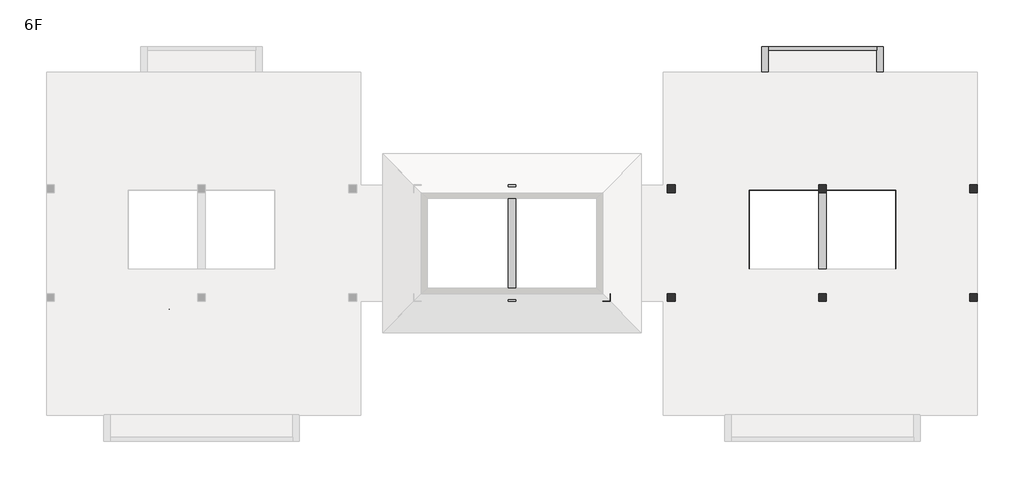
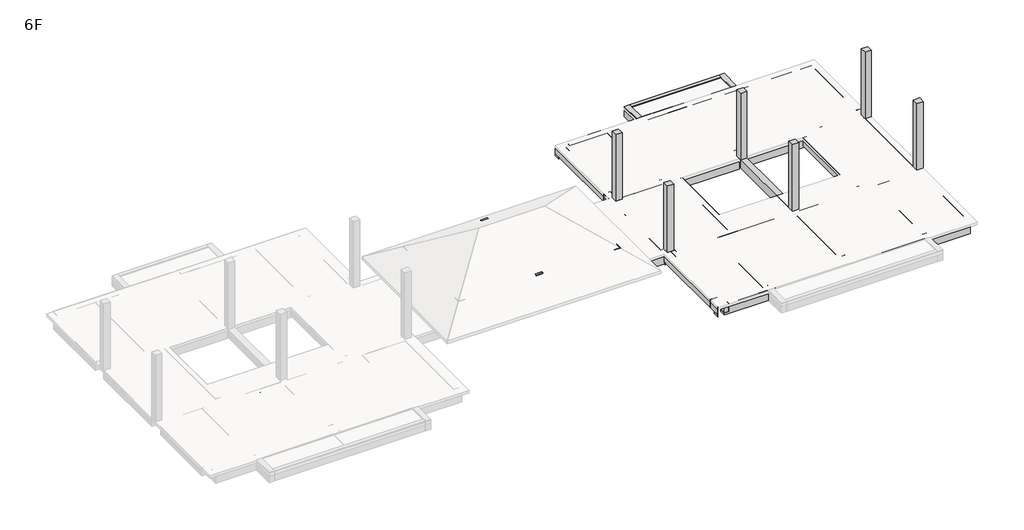
# One storey, part 2 of 2: 33 beams, 10 columns, 1 proxy.
"""IFC4 building model written with IfcOpenShell, lengths in millimetres."""

import ifcopenshell
import ifcopenshell.guid

model = None  # the IFC model being written
_history = None  # IfcOwnerHistory: only IFC2X3 demands one
_inside = {}  # id of a spatial element -> (the spatial element, [elements in it])
_under = {}  # id of a project, library or spatial element -> (it, [spatial elements below it])
_declared = {}  # id of a project -> (the project, [libraries it declares])
_typed = {}  # id of a type object -> (the type object, [elements of that type])
_made_of = {}  # id of a material, layer set ... -> (it, [elements and type objects made of it])


def new_model(schema):
    """Start an empty IFC model of exactly this schema.

    Asked for "IFC4X3", IfcOpenShell would pick the latest addendum, in which some entities
    have other attributes; the version numbers below select the first issue.
    IFC2X3 requires an IfcOwnerHistory on every rooted entity: one is made here for all.
    """
    global model, _history
    if schema == "IFC4X3":
        model = ifcopenshell.file(schema_version=(4, 3, 0, 0))
    else:
        model = ifcopenshell.file(schema=schema)
    _inside.clear()
    _under.clear()
    _declared.clear()
    _typed.clear()
    _made_of.clear()
    _history = None
    if model.schema == "IFC2X3":
        org = make("IfcOrganization", Name="unknown")
        user = make(
            "IfcPersonAndOrganization",
            ThePerson=make("IfcPerson", FamilyName="unknown"),
            TheOrganization=org,
        )
        app = make(
            "IfcApplication",
            ApplicationDeveloper=org,
            Version="unknown",
            ApplicationFullName="unknown",
            ApplicationIdentifier="unknown",
        )
        _history = make(
            "IfcOwnerHistory",
            OwningUser=user,
            OwningApplication=app,
            ChangeAction="ADDED",
            CreationDate=0,
        )
    return model


def make(cls, **values):
    """One entity of the class cls with the attributes given. An attribute that is None is left unset."""
    return model.create_entity(
        cls, **{name: value for name, value in values.items() if value is not None}
    )


def rooted(cls, **values):
    """An entity with a GlobalId (a new one), such as an element, a storey or a relation."""
    return make(cls, GlobalId=ifcopenshell.guid.new(), OwnerHistory=_history, **values)


def si_unit(unit_type, name, prefix=None):
    """IfcSIUnit, for example si_unit("LENGTHUNIT", "METRE", prefix="MILLI")."""
    return make("IfcSIUnit", UnitType=unit_type, Prefix=prefix, Name=name)


def assignment(units):
    """IfcUnitAssignment: the units of a project."""
    return None if units is None else make("IfcUnitAssignment", Units=units)


def point(xyz):
    """IfcCartesianPoint."""
    return None if xyz is None else make("IfcCartesianPoint", Coordinates=xyz)


def direction(xyz):
    """IfcDirection."""
    return None if xyz is None else make("IfcDirection", DirectionRatios=xyz)


def frame(location, z_axis=None, x_axis=None):
    """IfcAxis2Placement3D, a coordinate frame: its origin and axes. An axis left out is left unset."""
    return make(
        "IfcAxis2Placement3D",
        Location=point(location),
        Axis=direction(z_axis),
        RefDirection=direction(x_axis),
    )


def frame_2d(location, x_axis=None):
    """IfcAxis2Placement2D, a coordinate frame in the plane: its origin and x axis."""
    return make(
        "IfcAxis2Placement2D", Location=point(location), RefDirection=direction(x_axis)
    )


def origin():
    """The frame at (0, 0, 0) with its axes left unset."""
    return frame((0.0, 0.0, 0.0))


def origin_with_axes():
    """The frame at (0, 0, 0) with the z axis (0, 0, 1) and the x axis (1, 0, 0) written out."""
    return frame((0.0, 0.0, 0.0), z_axis=(0.0, 0.0, 1.0), x_axis=(1.0, 0.0, 0.0))


def place(relative_to, where):
    """IfcLocalPlacement: puts the frame where relative to a parent placement (None: the world)."""
    return make(
        "IfcLocalPlacement", PlacementRelTo=relative_to, RelativePlacement=where
    )


def context(
    kind, dimensions, precision=None, world=None, true_north=None, identifier=None
):
    """IfcGeometricRepresentationContext, for example the 3D "Model" context."""
    return make(
        "IfcGeometricRepresentationContext",
        ContextIdentifier=identifier,
        ContextType=kind,
        CoordinateSpaceDimension=dimensions,
        Precision=precision,
        WorldCoordinateSystem=world,
        TrueNorth=true_north,
    )


def project(units=None, contexts=None):
    """IfcProject with its units and contexts."""
    return rooted(
        "IfcProject",
        Name="project",
        RepresentationContexts=contexts,
        UnitsInContext=assignment(units),
    )


def spatial(cls, under=None, at=None, **own):
    """A site, building, storey or space (cls), placed at a placement, below another one or the project."""
    s = rooted(cls, ObjectPlacement=at, **own)
    if under is not None:
        _under.setdefault(under.id(), (under, []))[1].append(s)
    return s


def polyline(points):
    """IfcPolyline through the points."""
    return make("IfcPolyline", Points=[point(p) for p in points])


def circle_curve(where, radius):
    """IfcCircle in the frame where."""
    return make("IfcCircle", Position=where, Radius=radius)


def ellipse_curve(where, semi_axis1, semi_axis2):
    """IfcEllipse in the frame where."""
    return make(
        "IfcEllipse", Position=where, SemiAxis1=semi_axis1, SemiAxis2=semi_axis2
    )


def trimmed(basis, trim1, trim2, sense, master):
    """IfcTrimmedCurve: the piece of a basis curve between two trims."""
    return make(
        "IfcTrimmedCurve",
        BasisCurve=basis,
        Trim1=trim1,
        Trim2=trim2,
        SenseAgreement=sense,
        MasterRepresentation=master,
    )


def segment(curve, same_sense, transition):
    """IfcCompositeCurveSegment."""
    return make(
        "IfcCompositeCurveSegment",
        Transition=transition,
        SameSense=same_sense,
        ParentCurve=curve,
    )


def composite_curve(segments, self_intersect=None):
    """IfcCompositeCurve: segments joined end to end."""
    return make("IfcCompositeCurve", Segments=segments, SelfIntersect=self_intersect)


def outline(outer, holes=None, kind="AREA"):
    """IfcArbitraryClosedProfileDef: a profile drawn as a closed curve; with holes, ...WithVoids."""
    if holes is None:
        return make("IfcArbitraryClosedProfileDef", ProfileType=kind, OuterCurve=outer)
    return make(
        "IfcArbitraryProfileDefWithVoids",
        ProfileType=kind,
        OuterCurve=outer,
        InnerCurves=holes,
    )


def extrude(swept, where, along, depth):
    """IfcExtrudedAreaSolid: the profile swept, set in the frame where, extruded along a direction by depth."""
    return make(
        "IfcExtrudedAreaSolid",
        SweptArea=swept,
        Position=where,
        ExtrudedDirection=direction(along),
        Depth=depth,
    )


def faces_of(points, faces, orient=None, outer=None):
    """IfcFace entities. A face is a list of loops; a loop is a list of indices into points, from 0.

    orient and outer hold one flag for each loop. By default every Orientation is true, the
    first loop of a face is its IfcFaceOuterBound and the others are IfcFaceBound.
    """
    made = []
    for i, loops in enumerate(faces):
        bounds = []
        for j, loop in enumerate(loops):
            is_outer = j == 0 if outer is None else outer[i][j]
            bounds.append(
                make(
                    "IfcFaceOuterBound" if is_outer else "IfcFaceBound",
                    Bound=make("IfcPolyLoop", Polygon=[points[k] for k in loop]),
                    Orientation=True if orient is None else orient[i][j],
                )
            )
        made.append(make("IfcFace", Bounds=bounds))
    return made


def faceted_brep(points, faces, orient=None, outer=None, voids=None):
    """IfcFacetedBrep: a solid bounded by flat faces; with voids (closed shells), ...WithVoids."""
    shared = [point(p) for p in points]
    hull = make("IfcClosedShell", CfsFaces=faces_of(shared, faces, orient, outer))
    if voids is None:
        return make("IfcFacetedBrep", Outer=hull)
    return make(
        "IfcFacetedBrepWithVoids",
        Outer=hull,
        Voids=[
            make(cls, CfsFaces=faces_of(shared, fs, o, b)) for cls, fs, o, b in voids
        ],
    )


def shape(context_of_items, identifier, shape_type, items):
    """IfcShapeRepresentation: the items that make up one representation, for example the "Body"."""
    return make(
        "IfcShapeRepresentation",
        ContextOfItems=context_of_items,
        RepresentationIdentifier=identifier,
        RepresentationType=shape_type,
        Items=items,
    )


def source(mapping_origin, context_of_items, identifier, shape_type, items):
    """IfcRepresentationMap: a shape defined once, which mapped items show again and again."""
    return make(
        "IfcRepresentationMap",
        MappingOrigin=mapping_origin,
        MappedRepresentation=shape(context_of_items, identifier, shape_type, items),
    )


def transform(
    local_origin,
    x_axis=None,
    y_axis=None,
    z_axis=None,
    scale=None,
    scale2=None,
    scale3=None,
    uniform=True,
):
    """IfcCartesianTransformationOperator3D, or its non-uniform kind. x_axis, y_axis, z_axis: its Axis1, 2, 3."""
    if uniform:
        return make(
            "IfcCartesianTransformationOperator3D",
            Axis1=direction(x_axis),
            Axis2=direction(y_axis),
            LocalOrigin=point(local_origin),
            Scale=scale,
            Axis3=direction(z_axis),
        )
    return make(
        "IfcCartesianTransformationOperator3DnonUniform",
        Axis1=direction(x_axis),
        Axis2=direction(y_axis),
        LocalOrigin=point(local_origin),
        Scale=scale,
        Axis3=direction(z_axis),
        Scale2=scale2,
        Scale3=scale3,
    )


def mapped(mapping_source, mapping_target):
    """IfcMappedItem: shows the shape of a source again, moved by a transform."""
    return make(
        "IfcMappedItem", MappingSource=mapping_source, MappingTarget=mapping_target
    )


def made_of(thing, what):
    """Note that an element or type object is made of a material, layer set ...; save() writes the relation."""
    if what is not None:
        _made_of.setdefault(what.id(), (what, []))[1].append(thing)
    return thing


def element(
    cls,
    number,
    at=None,
    inside=None,
    cuts=None,
    type_object=None,
    material=None,
    context=None,
    identifier="Body",
    shape_type=None,
    held_by="IfcProductDefinitionShape",
    body=None,
    shapes=None,
    **own,
):
    """One element of the class cls, such as IfcWall. Its Tag is "e" and its number.

    at: its placement. inside: the storey or other place that contains it. cuts: it is an
    opening in that element (IfcRelVoidsElement). A single representation is given by context,
    identifier, shape_type and body (its items); several are given by shapes. held_by: the class
    of the entity that holds the representations. save() writes the other relations.
    """
    e = rooted(cls, Tag="e%d" % number, ObjectPlacement=at, **own)
    if body is not None:
        shapes = [shape(context, identifier, shape_type, body)]
    if shapes is not None:
        e.Representation = make(held_by, Representations=shapes)
    if inside is not None:
        _inside.setdefault(inside.id(), (inside, []))[1].append(e)
    if cuts is not None:
        rooted(
            "IfcRelVoidsElement", RelatingBuildingElement=cuts, RelatedOpeningElement=e
        )
    if type_object is not None:
        _typed.setdefault(type_object.id(), (type_object, []))[1].append(e)
    return made_of(e, material)


def aggregate(whole, parts):
    """IfcRelAggregates: a whole, such as a stair, and the parts it consists of."""
    return rooted("IfcRelAggregates", RelatingObject=whole, RelatedObjects=parts)


def save(model, path):
    """Write the relations noted so far, then the file.

    IfcRelAggregates (storeys below a building ...), IfcRelContainedInSpatialStructure (elements
    in a storey), IfcRelDefinesByType, IfcRelAssociatesMaterial and IfcRelDeclares: one each for
    every whole, place, type object, material and project.
    """
    for whole, parts in _under.values():
        aggregate(whole, parts)
    for where, things in _inside.values():
        rooted(
            "IfcRelContainedInSpatialStructure",
            RelatedElements=things,
            RelatingStructure=where,
        )
    for kind, things in _typed.values():
        rooted("IfcRelDefinesByType", RelatedObjects=things, RelatingType=kind)
    for what, things in _made_of.values():
        rooted("IfcRelAssociatesMaterial", RelatedObjects=things, RelatingMaterial=what)
    for by, libraries in _declared.values():
        rooted("IfcRelDeclares", RelatingContext=by, RelatedDefinitions=libraries)
    model.write(path)


def plane_surface(at):
    """IfcPlane: the flat surface through the origin of the frame at, square to its z axis."""
    return make("IfcPlane", Position=at)


def cylinder_surface(at, radius):
    """IfcCylindricalSurface: all points at the distance radius from the z axis of the frame at."""
    return make("IfcCylindricalSurface", Position=at, Radius=radius)


def revolved_surface(curve, axis_point, axis_direction):
    """IfcSurfaceOfRevolution: the curve turned about the line through axis_point along axis_direction."""
    return make(
        "IfcSurfaceOfRevolution",
        SweptCurve=make("IfcArbitraryOpenProfileDef", ProfileType="CURVE", Curve=curve),
        AxisPosition=make("IfcAxis1Placement", Location=point(axis_point), Axis=direction(axis_direction)),
    )


def advanced_brep(points, edges, surfaces, faces):
    """IfcAdvancedBrep: a solid bounded by faces that lie on surfaces and meet in shared edges.

    An edge is (start, end): straight between two places in points (the first is 0);
    or (start, end, curve); or (start, end, curve, False) where it runs against its curve.
    A face is (place in surfaces, loops), or (place, loops, False) where it looks against
    its surface's normal. A loop lists edges by number (the first is 1), with a minus sign
    where the edge is run from its end to its start. The first loop is the outer one.
    """
    corners = [point(p) for p in points]
    vertices = [make("IfcVertexPoint", VertexGeometry=c) for c in corners]
    made = []
    for start, end, *more in edges:
        made.append(
            make(
                "IfcEdgeCurve",
                EdgeStart=vertices[start],
                EdgeEnd=vertices[end],
                EdgeGeometry=more[0] if more else make("IfcPolyline", Points=[corners[start], corners[end]]),
                SameSense=more[1] if len(more) > 1 else True,
            )
        )
    hull = []
    for where, loops, *sense in faces:
        bounds = []
        for j, loop in enumerate(loops):
            ring = [make("IfcOrientedEdge", EdgeElement=made[abs(k) - 1], Orientation=k > 0) for k in loop]
            bounds.append(
                make(
                    "IfcFaceOuterBound" if j == 0 else "IfcFaceBound",
                    Bound=make("IfcEdgeLoop", EdgeList=ring),
                    Orientation=True,
                )
            )
        hull.append(make("IfcAdvancedFace", Bounds=bounds, FaceSurface=surfaces[where], SameSense=sense[0] if sense else True))
    return make("IfcAdvancedBrep", Outer=make("IfcClosedShell", CfsFaces=hull))


def m_support_metal_circular_m_support_metal_circular_a779fbb7(model_context):
    return source(origin(), model_context, "Body", "SolidModel", [
        advanced_brep(
        [(-6.0, 0.0, 0.0), (6.0, 0.0, 0.0), (-6.0, 0.0, -63.0), (6.0, 0.0, -63.0), (6.0, 12.0, -75.0), (-6.0, 12.0, -75.0), (-6.0, 63.0, -75.0), (6.0, 63.0, -75.0)],
        [
            (0, 1, circle_curve(origin_with_axes(), 6.0)),
            (1, 0, circle_curve(origin_with_axes(), 6.0)),
            (0, 2),
            (2, 3, circle_curve(frame((0.0, 0.0, -63.0), z_axis=(0.0, 0.0, 1.0), x_axis=(1.0, 0.0, 0.0)), 6.0)),
            (3, 1),
            (3, 2, circle_curve(frame((0.0, 0.0, -63.0), z_axis=(0.0, 0.0, 1.0), x_axis=(1.0, 0.0, 0.0)), 6.0)),
            (4, 3, circle_curve(frame((6.0, 12.0, -63.0), z_axis=(-1.0, 0.0, 0.0), x_axis=(0.0, -1.0, 0.0)), 12.0)),
            (2, 5, circle_curve(frame((-6.0, 12.0, -63.0), z_axis=(1.0, 0.0, 0.0), x_axis=(0.0, -1.0, 0.0)), 12.0)),
            (5, 4, circle_curve(frame((0.0, 12.0, -75.0), z_axis=(0.0, -1.0, 0.0), x_axis=(1.0, 0.0, 0.0)), 6.0)),
            (4, 5, circle_curve(frame((0.0, 12.0, -75.0), z_axis=(0.0, -1.0, 0.0), x_axis=(1.0, 0.0, 0.0)), 6.0)),
            (6, 7, circle_curve(frame((0.0, 63.0, -75.0), z_axis=(0.0, 1.0, 0.0), x_axis=(1.0, 0.0, 0.0)), 6.0)),
            (7, 6, circle_curve(frame((0.0, 63.0, -75.0), z_axis=(0.0, 1.0, 0.0), x_axis=(1.0, 0.0, 0.0)), 6.0)),
            (5, 6),
            (7, 4),
        ],
        [
            plane_surface(origin_with_axes()),
            cylinder_surface(origin_with_axes(), 6.0),
            revolved_surface(trimmed(ellipse_curve(frame((0.0, 0.0, -63.0), z_axis=(0.0, 0.0, 1.0), x_axis=(1.0, 0.0, 0.0)), 6.0, 6.0), [point((-6.0, 0.0, -63.0))], [point((6.0, 0.0, -63.0))], True, "CARTESIAN"), (0.0, 12.0, -63.0), (1.0, 0.0, 0.0)),
            revolved_surface(trimmed(ellipse_curve(frame((0.0, 0.0, -63.0), z_axis=(0.0, 0.0, 1.0), x_axis=(1.0, 0.0, 0.0)), 6.0, 6.0), [point((6.0, 0.0, -63.0))], [point((-6.0, 0.0, -63.0))], True, "CARTESIAN"), (0.0, 12.0, -63.0), (1.0, 0.0, 0.0)),
            plane_surface(frame((0.0, 63.0, -75.0), z_axis=(0.0, 1.0, 0.0), x_axis=(1.0, 0.0, 0.0))),
            cylinder_surface(frame((0.0, 12.0, -75.0), z_axis=(0.0, -1.0, 0.0), x_axis=(1.0, 0.0, 0.0)), 6.0),
        ],
        [
            (0, [[1, 2]]),
            (1, [[-1, 3, 4, 5]]),
            (1, [[-2, -5, 6, -3]]),
            (2, [[7, -4, 8, 9]]),
            (3, [[-8, -6, -7, 10]]),
            (4, [[11, 12]]),
            (5, [[-9, 13, -12, 14]]),
            (5, [[-10, -14, -11, -13]]),
        ],
    ),
        extrude(outline(composite_curve([segment(trimmed(circle_curve(frame_2d((-75.0, 0.0)), 25.0), [point((-75.0, -25.0))], [point((-75.0, 25.0))], False, "CARTESIAN"), True, "CONTINUOUS"), segment(trimmed(circle_curve(frame_2d((-75.0, 0.0)), 25.0), [point((-75.0, 25.0))], [point((-75.0, -25.0))], False, "CARTESIAN"), True, "CONTINUOUS")], self_intersect=False)), frame((0.0, 63.0, 0.0), z_axis=(0.0, 1.0, 0.0), x_axis=(0.0, 0.0, 1.0)), (0.0, 0.0, 1.0), 12.0),
    ])


model = new_model("IFC4")

# Units and contexts
model_context = context("Model", 3, world=origin())
ifc_project = project(units=[si_unit("LENGTHUNIT", "METRE", prefix="MILLI")], contexts=[model_context])

# Site, building, storey
site = spatial("IfcSite", under=ifc_project)
building = spatial("IfcBuilding", under=site)
storey = spatial("IfcBuildingStorey", under=building, Name="6F", Elevation=17230.0)

# Beams
placement = place(None, origin())
element("IfcBeam", 1, ObjectType="M_Concrete-Rectangular Beam : 150x500", at=placement, inside=storey, context=model_context, shape_type="SweptSolid", body=[
    extrude(outline(polyline([(31939.6333637, 14100.0000002), (31939.6333637, 13950.0000002), (27759.4337113, 13950.0000002), (27759.4337113, 14100.0000002), (31939.6333637, 14100.0000002)])), frame((0.0, 0.0, 16730.0), z_axis=(0.0, 0.0, 1.0), x_axis=(1.0, 0.0, 0.0)), (0.0, 0.0, 1.0), 500.0),
])
element("IfcBeam", 2, ObjectType="M_Concrete-Rectangular Beam : 250x400", at=placement, inside=storey, context=model_context, shape_type="Brep", body=[
    faceted_brep([(32930.0000108, 8549.9999993, 17230.0), (32680.0000108, 8549.9999993, 17230.0), (32680.0000108, 4449.9999998, 17230.0), (32930.0000108, 4449.9999998, 17230.0), (32930.0000108, 8549.9999993, 16830.0), (32930.0000108, 4449.9999998, 16830.0), (32680.0000108, 8549.9999993, 16830.0), (32680.0000108, 4449.9999998, 16830.0), (32680.0000108, 8549.9999993, 17088.8582284)], [[[0, 1, 2, 3]], [[4, 0, 3, 5]], [[6, 4, 5, 7]], [[1, 8, 6, 7, 2]], [[1, 0, 4, 6, 8]], [[3, 2, 7, 5]]]),
])
element("IfcBeam", 3, ObjectType="M_Concrete-Rectangular Beam : 250x400", at=placement, inside=storey, context=model_context, shape_type="SweptSolid", body=[
    extrude(outline(polyline([(21399.9824991, 8449.9999993), (21649.9824991, 8449.9999993), (21649.9824991, 4549.9999902), (21399.9824991, 4549.9999902), (21399.9824991, 8449.9999993)])), frame((0.0, 0.0, 16830.0), z_axis=(0.0, 0.0, 1.0), x_axis=(1.0, 0.0, 0.0)), (0.0, 0.0, 1.0), 400.0),
])
element("IfcBeam", 4, ObjectType="M_Concrete-Rectangular Beam : 250x400", at=placement, inside=storey, context=model_context, shape_type="Brep", body=[
    faceted_brep([(27020.000004, 8549.9999993, 17230.0), (26770.000004, 8549.9999993, 17230.0), (26770.000004, 4449.9999998, 17230.0), (27020.000004, 4449.9999998, 17230.0), (27020.000004, 8549.9999993, 16830.0), (27020.000004, 8549.9999993, 17088.8582239), (27020.000004, 4449.9999998, 16830.0), (26770.000004, 8549.9999993, 16830.0), (26770.000004, 4449.9999998, 16830.0)], [[[0, 1, 2, 3]], [[4, 5, 0, 3, 6]], [[7, 4, 6, 8]], [[1, 7, 8, 2]], [[1, 0, 5, 4, 7]], [[3, 2, 8, 6]]]),
])
element("IfcBeam", 5, ObjectType="M_Concrete-Rectangular Beam : 250x400", at=placement, inside=storey, context=model_context, shape_type="SweptSolid", body=[
    extrude(outline(polyline([(25965.079965, 12800.0000001), (26215.079965, 12800.0000001), (26215.079965, 8849.9999993), (25965.079965, 8849.9999993), (25965.079965, 12800.0000001)])), frame((0.0, 0.0, 16830.0), z_axis=(0.0, 0.0, 1.0), x_axis=(1.0, 0.0, 0.0)), (0.0, 0.0, 1.0), 400.0),
])
element("IfcBeam", 6, ObjectType="M_Concrete-Rectangular Beam : 250x400", at=placement, inside=storey, context=model_context, shape_type="SweptSolid", body=[
    extrude(outline(polyline([(25965.079965, 4149.9999998), (26215.079965, 4149.9999998), (26215.079965, 199.9999987), (25965.079965, 199.9999987), (25965.079965, 4149.9999998)])), frame((0.0, 0.0, 16830.0), z_axis=(0.0, 0.0, 1.0), x_axis=(1.0, 0.0, 0.0)), (0.0, 0.0, 1.0), 400.0),
])
element("IfcBeam", 7, ObjectType="M_Concrete-Rectangular Beam : 250x400", at=placement, inside=storey, context=model_context, shape_type="SweptSolid", body=[
    extrude(outline(polyline([(33485.0000061, 12800.0000001), (33735.0000061, 12800.0000001), (33735.0000061, 8849.9999993), (33485.0000061, 8849.9999993), (33485.0000061, 12800.0000001)])), frame((0.0, 0.0, 16830.0), z_axis=(0.0, 0.0, 1.0), x_axis=(1.0, 0.0, 0.0)), (0.0, 0.0, 1.0), 400.0),
])
element("IfcBeam", 8, ObjectType="M_Concrete-Rectangular Beam : 250x400", at=placement, inside=storey, context=model_context, shape_type="SweptSolid", body=[
    extrude(outline(polyline([(33485.0000061, 4149.9999998), (33735.0000061, 4149.9999998), (33735.0000061, 199.9999987), (33485.0000061, 199.9999987), (33485.0000061, 4149.9999998)])), frame((0.0, 0.0, 16830.0), z_axis=(0.0, 0.0, 1.0), x_axis=(1.0, 0.0, 0.0)), (0.0, 0.0, 1.0), 400.0),
])
element("IfcBeam", 9, ObjectType="M_Concrete-Rectangular Beam : 250x400", at=placement, inside=storey, context=model_context, shape_type="SweptSolid", body=[
    extrude(outline(polyline([(18180.0, 21379.9824991), (17780.0, 21379.9824991), (17780.0, 21629.9824991), (18098.9682373, 21629.9824991), (18180.0, 21508.4286852), (18180.0, 21379.9824991)])), frame((0.0, 4550.0000005, 0.0), z_axis=(0.0, 1.0, 0.0), x_axis=(0.0, 0.0, 1.0)), (0.0, 0.0, 1.0), 3899.9999997),
])
element("IfcBeam", 10, ObjectType="M_Concrete-Rectangular Beam : 250x400", at=placement, inside=storey, context=model_context, shape_type="SweptSolid", body=[
    extrude(outline(polyline([(8724.9999993, 17780.0), (8474.9999993, 17780.0), (8474.9999993, 18180.0), (8608.4366337, 18180.0), (8724.9999993, 18102.2891349), (8724.9999993, 17780.0)])), frame((14350.0174936, 0.0, 0.0), z_axis=(1.0, 0.0, 0.0), x_axis=(0.0, 1.0, 0.0)), (0.0, 0.0, 1.0), 3349.7492755),
    extrude(outline(polyline([(8724.9999993, 17780.0), (8474.9999993, 17780.0), (8474.9999993, 18180.0), (8608.4366337, 18180.0), (8724.9999993, 18102.2891349), (8724.9999993, 17780.0)])), frame((17999.7667691, 0.0, 0.0), z_axis=(1.0, 0.0, 0.0), x_axis=(0.0, 1.0, 0.0)), (0.0, 0.0, 1.0), 3350.0),
])
element("IfcBeam", 11, ObjectType="M_Concrete-Rectangular Beam : 250x400", at=placement, inside=storey, context=model_context, shape_type="SweptSolid", body=[
    extrude(outline(polyline([(4524.9999902, 17780.0), (4274.9999902, 17780.0), (4274.9999902, 18102.6390219), (4391.0385385, 18180.0), (4524.9999902, 18180.0), (4524.9999902, 17780.0)])), frame((17999.7667691, 0.0, 0.0), z_axis=(1.0, 0.0, 0.0), x_axis=(0.0, 1.0, 0.0)), (0.0, 0.0, 1.0), 3350.0),
    extrude(outline(polyline([(4524.9999902, 18180.0), (4524.9999902, 17780.0), (4274.9999902, 17780.0), (4274.9999902, 18102.6390219), (4391.0385385, 18180.0), (4524.9999902, 18180.0)])), frame((14350.0174936, 0.0, 0.0), z_axis=(1.0, 0.0, 0.0), x_axis=(0.0, 1.0, 0.0)), (0.0, 0.0, 1.0), 3349.7492755),
])
element("IfcBeam", 12, ObjectType="M_Concrete-Rectangular Beam : 250x500", at=placement, inside=storey, context=model_context, shape_type="Brep", body=[
    faceted_brep([(32189.6333637, 14100.0000002, 17230.0), (31939.6333637, 14100.0000002, 17230.0), (31939.6333637, 13950.0000002, 17230.0), (31939.6333637, 13100.0000001, 17230.0), (32189.6333637, 13100.0000001, 17230.0), (31939.6333637, 14100.0000002, 16730.0), (31939.6333637, 13950.0000002, 16730.0), (31939.6333637, 13100.0000001, 16730.0), (32189.6333637, 14100.0000002, 16730.0), (32189.6333637, 13100.0000001, 16730.0)], [[[0, 1, 2, 3, 4]], [[1, 5, 6, 7, 3, 2]], [[5, 8, 9, 7, 6]], [[8, 0, 4, 9]], [[1, 0, 8, 5]], [[4, 3, 7, 9]]]),
])
element("IfcBeam", 13, ObjectType="M_Concrete-Rectangular Beam : 250x500", at=placement, inside=storey, context=model_context, shape_type="Brep", body=[
    faceted_brep([(27759.4337113, 14100.0000002, 17230.0), (27509.4337113, 14100.0000002, 17230.0), (27509.4337113, 13100.0000001, 17230.0), (27759.4337113, 13100.0000001, 17230.0), (27759.4337113, 13950.0000002, 17230.0), (27509.4337113, 14100.0000002, 16730.0), (27509.4337113, 13100.0000001, 16730.0), (27759.4337113, 14100.0000002, 16730.0), (27759.4337113, 13950.0000002, 16730.0), (27759.4337113, 13100.0000001, 16730.0)], [[[0, 1, 2, 3, 4]], [[1, 5, 6, 2]], [[5, 7, 8, 9, 6]], [[7, 0, 4, 3, 9, 8]], [[1, 0, 7, 5]], [[3, 2, 6, 9]]]),
])
element("IfcBeam", 14, ObjectType="M_Concrete-Rectangular Beam : 300x400", at=placement, inside=storey, context=model_context, shape_type="Brep", body=[
    faceted_brep([(18000.0000046, 8450.0000002, 17230.0), (17700.0000046, 8449.9999993, 17230.0), (17700.0000046, 4549.9999902, 17230.0), (18000.0000046, 4549.9999902, 17230.0), (17700.0000046, 8449.9999993, 16830.0), (17700.0000046, 4549.9999902, 16830.0), (18000.0000046, 8450.0000002, 16830.0), (18000.0000046, 4549.9999902, 16830.0)], [[[0, 1, 2, 3]], [[1, 4, 5, 2]], [[4, 6, 7, 5]], [[3, 7, 6, 0]], [[0, 6, 4, 1]], [[3, 2, 5, 7]]]),
])
element("IfcBeam", 15, ObjectType="M_Concrete-Rectangular Beam : 300x400", at=placement, inside=storey, context=model_context, shape_type="SweptSolid", body=[
    extrude(outline(polyline([(30000.0000031, 9150.0000002), (29700.0000031, 9150.0000002), (29700.0000031, 12500.0000005), (30000.0000031, 12500.0000005), (30000.0000031, 9150.0000002)])), frame((0.0, 0.0, 16830.0), z_axis=(0.0, 0.0, 1.0), x_axis=(1.0, 0.0, 0.0)), (0.0, 0.0, 1.0), 400.0),
])
element("IfcBeam", 16, ObjectType="M_Concrete-Rectangular Beam : 300x400", at=placement, inside=storey, context=model_context, shape_type="SweptSolid", body=[
    extrude(outline(polyline([(30000.0000031, 4550.0000002), (29700.0000031, 4550.0000002), (29700.0000031, 8450.0000002), (30000.0000031, 8450.0000002), (30000.0000031, 4550.0000002)])), frame((0.0, 0.0, 16830.0), z_axis=(0.0, 0.0, 1.0), x_axis=(1.0, 0.0, 0.0)), (0.0, 0.0, 1.0), 400.0),
])
element("IfcBeam", 17, ObjectType="M_Concrete-Rectangular Beam : 300x400", at=placement, inside=storey, context=model_context, shape_type="SweptSolid", body=[
    extrude(outline(polyline([(30000.0000031, 500.0), (29700.0000031, 500.0), (29700.0000031, 3850.0000002), (30000.0000031, 3850.0000002), (30000.0000031, 500.0)])), frame((0.0, 0.0, 16830.0), z_axis=(0.0, 0.0, 1.0), x_axis=(1.0, 0.0, 0.0)), (0.0, 0.0, 1.0), 400.0),
])
element("IfcBeam", 18, ObjectType="M_Concrete-Rectangular Beam : 300x400", at=placement, inside=storey, context=model_context, shape_type="SweptSolid", body=[
    extrude(outline(polyline([(35835.035019, 9150.0000002), (35535.035019, 9150.0000002), (35535.035019, 12500.0000005), (35835.035019, 12500.0000005), (35835.035019, 9150.0000002)])), frame((0.0, 0.0, 16830.0), z_axis=(0.0, 0.0, 1.0), x_axis=(1.0, 0.0, 0.0)), (0.0, 0.0, 1.0), 400.0),
])
element("IfcBeam", 19, ObjectType="M_Concrete-Rectangular Beam : 300x400", at=placement, inside=storey, context=model_context, shape_type="SweptSolid", body=[
    extrude(outline(polyline([(35835.035019, 4550.0000002), (35535.035019, 4550.0000002), (35535.035019, 8450.0000002), (35835.035019, 8450.0000002), (35835.035019, 4550.0000002)])), frame((0.0, 0.0, 16830.0), z_axis=(0.0, 0.0, 1.0), x_axis=(1.0, 0.0, 0.0)), (0.0, 0.0, 1.0), 400.0),
])
element("IfcBeam", 20, ObjectType="M_Concrete-Rectangular Beam : 300x400", at=placement, inside=storey, context=model_context, shape_type="SweptSolid", body=[
    extrude(outline(polyline([(35835.035019, 500.0), (35535.035019, 500.0), (35535.035019, 3850.0000002), (35835.035019, 3850.0000002), (35835.035019, 500.0)])), frame((0.0, 0.0, 16830.0), z_axis=(0.0, 0.0, 1.0), x_axis=(1.0, 0.0, 0.0)), (0.0, 0.0, 1.0), 400.0),
])
element("IfcBeam", 21, ObjectType="M_Concrete-Rectangular Beam : 300x500", at=placement, inside=storey, context=model_context, shape_type="Brep", body=[
    faceted_brep([(24199.5160441, 8449.9999993, 17230.0), (24199.5160441, 8549.9999993, 17230.0), (24199.5160441, 8749.9999993, 17230.0), (23999.9649972, 8749.9999993, 17230.0), (23999.9649972, 8449.9999993, 17230.0), (24199.5160441, 8449.9999993, 16730.0), (24199.5160441, 8449.9999993, 16830.0), (23999.9649972, 8449.9999993, 16730.0), (24199.5160441, 8749.9999993, 16730.0), (24199.5160441, 8549.9999993, 16730.0), (23999.9649972, 8749.9999993, 16730.0), (24199.5160441, 8749.9999993, 16830.0), (23999.9649972, 8749.9999993, 16830.0)], [[[0, 1, 2, 3, 4]], [[5, 6, 0, 4, 7]], [[8, 9, 5, 7, 10]], [[2, 11, 8, 10, 12, 3]], [[2, 1, 0, 6, 5, 9, 8, 11]], [[4, 3, 12, 10, 7]]]),
    faceted_brep([(17999.9649983, 8449.9999993, 17230.0), (17999.9649983, 8749.9999993, 17230.0), (17999.9649983, 8749.9999993, 16730.0), (17999.9649983, 8449.9999993, 16730.0), (23699.9649972, 8749.9999993, 17230.0), (23699.9649972, 8449.9999993, 17230.0), (23699.9649972, 8449.9999993, 16730.0), (23699.9649972, 8749.9999993, 16730.0), (23699.9649972, 8749.9999993, 16830.0), (21399.9824991, 8449.9999993, 17230.0), (21649.9824991, 8449.9999993, 17230.0), (23699.5160441, 8449.9999993, 17230.0), (23699.5160441, 8749.9999993, 17230.0), (23699.5160441, 8749.9999993, 16730.0)], [[[0, 1, 2, 3]], [[4, 5, 6, 7, 8]], [[1, 0, 9, 10, 11, 5, 4, 12]], [[0, 3, 6, 5, 11, 10, 9]], [[3, 2, 13, 7, 6]], [[2, 1, 12, 4, 8, 7, 13]]]),
])
element("IfcBeam", 22, ObjectType="M_Concrete-Rectangular Beam : 300x500", at=placement, inside=storey, context=model_context, shape_type="Brep", body=[
    faceted_brep([(24199.5160441, 4249.9999902, 17230.0), (24199.5160441, 4449.9999998, 17230.0), (24199.5160441, 4549.9999902, 17230.0), (24000.0000047, 4549.9999902, 17230.0), (24000.0000047, 4249.9999902, 17230.0), (24199.5160441, 4249.9999902, 16730.0), (24199.5160441, 4249.9999902, 16830.0), (24000.0000047, 4249.9999902, 16830.0), (24000.0000047, 4249.9999902, 16730.0), (24199.5160441, 4549.9999902, 16730.0), (24199.5160441, 4449.9999998, 16730.0), (24000.0000047, 4549.9999902, 16730.0), (24199.5160441, 4549.9999902, 16830.0)], [[[0, 1, 2, 3, 4]], [[5, 6, 0, 4, 7, 8]], [[9, 10, 5, 8, 11]], [[2, 12, 9, 11, 3]], [[2, 1, 0, 6, 5, 10, 9, 12]], [[4, 3, 11, 8, 7]]]),
    faceted_brep([(18000.0000058, 4249.9999902, 17230.0), (18000.0000058, 4549.9999902, 17230.0), (18000.0000058, 4549.9999902, 16730.0), (18000.0000058, 4249.9999902, 16730.0), (23700.0000047, 4549.9999902, 17230.0), (23700.0000047, 4249.9999902, 17230.0), (23700.0000047, 4249.9999902, 16830.0), (23700.0000047, 4249.9999902, 16730.0), (23700.0000047, 4549.9999902, 16730.0), (23699.5160441, 4249.9999902, 17230.0), (23699.5160441, 4549.9999902, 17230.0), (21649.9824991, 4549.9999902, 17230.0), (21399.9824991, 4549.9999902, 17230.0), (23699.5160441, 4249.9999902, 16730.0)], [[[0, 1, 2, 3]], [[4, 5, 6, 7, 8]], [[1, 0, 9, 5, 4, 10, 11, 12]], [[0, 3, 13, 7, 6, 5, 9]], [[3, 2, 8, 7, 13]], [[2, 1, 12, 11, 10, 4, 8]]]),
])
element("IfcBeam", 23, ObjectType="M_Concrete-Rectangular Beam : 300x500", at=placement, inside=storey, context=model_context, shape_type="Brep", body=[
    faceted_brep([(24199.5160441, 13100.0000001, 17230.0), (24199.5160441, 12800.0000001, 17230.0), (25965.079965, 12800.0000001, 17230.0), (26215.079965, 12800.0000001, 17230.0), (29700.0000039, 12800.0000001, 17230.0), (29700.0000039, 13100.0000001, 17230.0), (27759.4337113, 13100.0000001, 17230.0), (27509.4337113, 13100.0000001, 17230.0), (24199.5160441, 12800.0000001, 16830.0), (24000.0000047, 12800.0000001, 16830.0), (24000.0000047, 12800.0000001, 16730.0), (29700.0000039, 12800.0000001, 16730.0), (29700.0000039, 13100.0000001, 16730.0), (24000.0000047, 13100.0000001, 16730.0), (27509.4337113, 13100.0000001, 16730.0), (27759.4337113, 13100.0000001, 16730.0), (24000.0000047, 13100.0000001, 16830.0), (24199.5160441, 13100.0000001, 16830.0)], [[[0, 1, 2, 3, 4, 5, 6, 7]], [[1, 8, 9, 10, 11, 4, 3, 2]], [[12, 11, 10, 13, 14, 15]], [[5, 12, 15, 14, 13, 16, 17, 0, 7, 6]], [[8, 17, 16, 9]], [[1, 0, 17, 8]], [[5, 4, 11, 12]], [[10, 9, 16, 13]]]),
    faceted_brep([(23699.5160441, 13100.0000001, 16730.0), (23699.5160441, 12800.0000001, 16730.0), (23699.5160441, 12800.0000001, 16830.0), (23699.5160441, 13100.0000001, 16830.0), (23700.0000047, 12800.0000001, 16830.0), (23700.0000047, 12800.0000001, 16730.0), (23700.0000047, 13100.0000001, 16730.0), (23700.0000047, 13100.0000001, 16830.0)], [[[0, 1, 2, 3]], [[4, 5, 6, 7]], [[2, 1, 5, 4]], [[1, 0, 6, 5]], [[0, 3, 7, 6]], [[3, 2, 4, 7]]]),
])
element("IfcBeam", 24, ObjectType="M_Concrete-Rectangular Beam : 300x500", at=placement, inside=storey, context=model_context, shape_type="Brep", body=[
    faceted_brep([(29699.9649964, 8549.9999993, 17230.0), (29699.9649964, 8849.9999993, 17230.0), (26215.079965, 8849.9999993, 17230.0), (25965.079965, 8849.9999993, 17230.0), (24199.5160441, 8849.9999993, 17230.0), (24199.5160441, 8749.9999993, 17230.0), (24199.5160441, 8549.9999993, 17230.0), (26770.000004, 8549.9999993, 17230.0), (27020.000004, 8549.9999993, 17230.0), (29699.9649964, 8549.9999993, 16730.0), (24199.5160441, 8549.9999993, 16730.0), (29699.9649964, 8849.9999993, 16730.0), (24199.5160441, 8749.9999993, 16730.0), (23999.9649972, 8749.9999993, 16730.0), (23999.9649972, 8849.9999993, 16730.0), (23999.9649972, 8849.9999993, 16830.0), (24199.5160441, 8849.9999993, 16830.0), (23999.9649972, 8749.9999993, 16830.0), (24199.5160441, 8749.9999993, 16830.0)], [[[0, 1, 2, 3, 4, 5, 6, 7, 8]], [[9, 0, 8, 7, 6, 10]], [[11, 9, 10, 12, 13, 14]], [[1, 11, 14, 15, 16, 4, 3, 2]], [[15, 14, 13, 17]], [[4, 16, 18, 12, 10, 6, 5]], [[1, 0, 9, 11]], [[16, 15, 17, 18]], [[12, 18, 17, 13]]]),
    faceted_brep([(23699.9649972, 8849.9999993, 16830.0), (23699.5160441, 8849.9999993, 16830.0), (23699.5160441, 8749.9999993, 16830.0), (23699.9649972, 8749.9999993, 16830.0), (23699.5160441, 8849.9999993, 16730.0), (23699.5160441, 8749.9999993, 16730.0), (23699.9649972, 8849.9999993, 16730.0), (23699.9649972, 8749.9999993, 16730.0)], [[[0, 1, 2, 3]], [[1, 4, 5, 2]], [[6, 0, 3, 7]], [[4, 6, 7, 5]], [[6, 4, 1, 0]], [[3, 2, 5, 7]]]),
])
element("IfcBeam", 25, ObjectType="M_Concrete-Rectangular Beam : 300x500", at=placement, inside=storey, context=model_context, shape_type="Brep", body=[
    faceted_brep([(29700.0000039, 4149.9999998, 17230.0), (29700.0000039, 4449.9999998, 17230.0), (27020.000004, 4449.9999998, 17230.0), (26770.000004, 4449.9999998, 17230.0), (24199.5160441, 4449.9999998, 17230.0), (24199.5160441, 4249.9999902, 17230.0), (24199.5160441, 4149.9999998, 17230.0), (25965.079965, 4149.9999998, 17230.0), (26215.079965, 4149.9999998, 17230.0), (24199.5160441, 4149.9999998, 16830.0), (24000.0000047, 4149.9999998, 16830.0), (24000.0000047, 4149.9999998, 16730.0), (29700.0000039, 4149.9999998, 16730.0), (29700.0000039, 4449.9999998, 16730.0), (24000.0000047, 4249.9999902, 16730.0), (24199.5160441, 4249.9999902, 16730.0), (24199.5160441, 4449.9999998, 16730.0), (24199.5160441, 4249.9999902, 16830.0), (24000.0000047, 4249.9999902, 16830.0)], [[[0, 1, 2, 3, 4, 5, 6, 7, 8]], [[6, 9, 10, 11, 12, 0, 8, 7]], [[13, 12, 11, 14, 15, 16]], [[1, 13, 16, 4, 3, 2]], [[9, 6, 5, 4, 16, 15, 17]], [[10, 9, 17, 18]], [[11, 10, 18, 14]], [[1, 0, 12, 13]], [[17, 15, 14, 18]]]),
    faceted_brep([(23699.5160441, 4149.9999998, 16730.0), (23699.5160441, 4149.9999998, 16830.0), (23699.5160441, 4249.9999902, 16830.0), (23699.5160441, 4249.9999902, 16730.0), (23700.0000047, 4149.9999998, 16830.0), (23700.0000047, 4149.9999998, 16730.0), (23700.0000047, 4249.9999902, 16730.0), (23700.0000047, 4249.9999902, 16830.0)], [[[0, 1, 2, 3]], [[4, 5, 6, 7]], [[1, 0, 5, 4]], [[5, 0, 3, 6]], [[1, 4, 7, 2]], [[3, 2, 7, 6]]]),
])
element("IfcBeam", 26, ObjectType="M_Concrete-Rectangular Beam : 300x500", at=placement, inside=storey, context=model_context, shape_type="Brep", body=[
    faceted_brep([(24199.5160441, 199.9999987, 17230.0), (24199.5160441, -100.0000013, 17230.0), (26070.012858, -100.0000013, 17230.0), (26320.012858, -100.0000013, 17230.0), (29700.0000039, -100.0000013, 17230.0), (29700.0000039, 199.9999987, 17230.0), (26215.079965, 199.9999987, 17230.0), (25965.079965, 199.9999987, 17230.0), (24000.0000047, -100.0000013, 16830.0), (24000.0000047, -100.0000013, 16730.0), (26070.012858, -100.0000013, 16730.0), (26320.012858, -100.0000013, 16730.0), (29700.0000039, -100.0000013, 16730.0), (24199.5160441, -100.0000013, 16830.0), (24000.0000047, 199.9999987, 16730.0), (29700.0000039, 199.9999987, 16730.0), (24199.5160441, 199.9999987, 16830.0), (24000.0000047, 199.9999987, 16830.0)], [[[0, 1, 2, 3, 4, 5, 6, 7]], [[8, 9, 10, 11, 12, 4, 3, 2, 1, 13]], [[9, 14, 15, 12, 11, 10]], [[16, 0, 7, 6, 5, 15, 14, 17]], [[1, 0, 16, 13]], [[17, 8, 13, 16]], [[9, 8, 17, 14]], [[5, 4, 12, 15]]]),
    faceted_brep([(23699.5160441, 199.9999987, 16730.0), (23699.5160441, -100.0000013, 16730.0), (23699.5160441, -100.0000013, 16830.0), (23699.5160441, 199.9999987, 16830.0), (23700.0000047, -100.0000013, 16830.0), (23700.0000047, -100.0000013, 16730.0), (23700.0000047, 199.9999987, 16730.0), (23700.0000047, 199.9999987, 16830.0)], [[[0, 1, 2, 3]], [[4, 5, 6, 7]], [[2, 1, 5, 4]], [[1, 0, 6, 5]], [[0, 3, 7, 6]], [[3, 2, 4, 7]]]),
])
element("IfcBeam", 27, ObjectType="M_Concrete-Rectangular Beam : 300x500", at=placement, inside=storey, context=model_context, shape_type="Brep", body=[
    faceted_brep([(30000.0000039, 13100.0000001, 17230.0), (30000.0000039, 12800.0000001, 17230.0), (33485.0000061, 12800.0000001, 17230.0), (33735.0000061, 12800.0000001, 17230.0), (35535.035019, 12800.0000001, 17230.0), (35535.035019, 13100.0000001, 17230.0), (32189.6333637, 13100.0000001, 17230.0), (31939.6333637, 13100.0000001, 17230.0), (30000.0000039, 12800.0000001, 16730.0), (35535.035019, 12800.0000001, 16730.0), (30000.0000039, 13100.0000001, 16730.0), (31939.6333637, 13100.0000001, 16730.0), (32189.6333637, 13100.0000001, 16730.0), (35535.035019, 13100.0000001, 16730.0)], [[[0, 1, 2, 3, 4, 5, 6, 7]], [[1, 8, 9, 4, 3, 2]], [[8, 10, 11, 12, 13, 9]], [[10, 0, 7, 6, 5, 13, 12, 11]], [[1, 0, 10, 8]], [[5, 4, 9, 13]]]),
])
element("IfcBeam", 28, ObjectType="M_Concrete-Rectangular Beam : 300x500", at=placement, inside=storey, context=model_context, shape_type="Brep", body=[
    faceted_brep([(29999.9649964, 8849.9999993, 17230.0), (29999.9649964, 8549.9999993, 17230.0), (32680.0000108, 8549.9999993, 17230.0), (32930.0000108, 8549.9999993, 17230.0), (35535.0000115, 8549.9999993, 17230.0), (35535.0000115, 8849.9999993, 17230.0), (33735.0000061, 8849.9999993, 17230.0), (33485.0000061, 8849.9999993, 17230.0), (29999.9649964, 8549.9999993, 16730.0), (35535.0000115, 8549.9999993, 16730.0), (29999.9649964, 8849.9999993, 16730.0), (35535.0000115, 8849.9999993, 16730.0)], [[[0, 1, 2, 3, 4, 5, 6, 7]], [[1, 8, 9, 4, 3, 2]], [[8, 10, 11, 9]], [[10, 0, 7, 6, 5, 11]], [[1, 0, 10, 8]], [[5, 4, 9, 11]]]),
])
element("IfcBeam", 29, ObjectType="M_Concrete-Rectangular Beam : 300x500", at=placement, inside=storey, context=model_context, shape_type="Brep", body=[
    faceted_brep([(30000.0000031, 4449.9999998, 17230.0), (30000.0000031, 4149.9999998, 17230.0), (33485.0000061, 4149.9999998, 17230.0), (33735.0000061, 4149.9999998, 17230.0), (35535.035019, 4149.9999998, 17230.0), (35535.035019, 4449.9999998, 17230.0), (32930.0000108, 4449.9999998, 17230.0), (32680.0000108, 4449.9999998, 17230.0), (30000.0000039, 4149.9999998, 16730.0), (35535.035019, 4149.9999998, 16730.0), (30000.0000039, 4449.9999998, 16730.0), (35535.035019, 4449.9999998, 16730.0)], [[[0, 1, 2, 3, 4, 5, 6, 7]], [[1, 8, 9, 4, 3, 2]], [[8, 10, 11, 9]], [[10, 0, 7, 6, 5, 11]], [[1, 0, 10, 8]], [[5, 4, 9, 11]]]),
])
element("IfcBeam", 30, ObjectType="M_Concrete-Rectangular Beam : 300x500", at=placement, inside=storey, context=model_context, shape_type="Brep", body=[
    faceted_brep([(30000.0000039, 199.9999987, 17230.0), (30000.0000039, -100.0000013, 17230.0), (33380.0128581, -100.0000013, 17230.0), (33630.0128581, -100.0000013, 17230.0), (35535.035019, -100.0000013, 17230.0), (35535.035019, 199.9999987, 17230.0), (33735.0000061, 199.9999987, 17230.0), (33485.0000061, 199.9999987, 17230.0), (30000.0000039, -100.0000013, 16730.0), (33380.0128581, -100.0000013, 16730.0), (33630.0128581, -100.0000013, 16730.0), (35535.035019, -100.0000013, 16730.0), (30000.0000039, 199.9999987, 16730.0), (35535.035019, 199.9999987, 16730.0)], [[[0, 1, 2, 3, 4, 5, 6, 7]], [[1, 8, 9, 10, 11, 4, 3, 2]], [[8, 12, 13, 11, 10, 9]], [[12, 0, 7, 6, 5, 13]], [[1, 0, 12, 8]], [[5, 4, 11, 13]]]),
])
element("IfcBeam", 31, ObjectType="M_Concrete-Rectangular Beam : 500x400", at=placement, inside=storey, context=model_context, shape_type="Brep", body=[
    faceted_brep([(23999.9649972, 9150.0000002, 17230.0), (23999.9649972, 8749.9999993, 17230.0), (24199.5160441, 8749.9999993, 17230.0), (24199.5160441, 8849.9999993, 17230.0), (24199.5160441, 12800.0000001, 17230.0), (24199.5160441, 13100.0000001, 17230.0), (24000.0000047, 13100.0000001, 17230.0), (24000.0000047, 12500.0000005, 17230.0), (23700.0000047, 12500.0000005, 17230.0), (23700.0000047, 13100.0000001, 17230.0), (23699.5160441, 13100.0000001, 17230.0), (23699.5160441, 8749.9999993, 17230.0), (23699.9649972, 8749.9999993, 17230.0), (23699.9649972, 9150.0000002, 17230.0), (23699.5160441, 8749.9999993, 16830.0), (23699.5160441, 13100.0000001, 16830.0), (23699.5160441, 12800.0000001, 16830.0), (23699.5160441, 8849.9999993, 16830.0), (23999.9649972, 8749.9999993, 16830.0), (23999.9649972, 8849.9999993, 16830.0), (23999.9649972, 9150.0000002, 16830.0), (23699.9649972, 9150.0000002, 16830.0), (23699.9649972, 8849.9999993, 16830.0), (23699.9649972, 8749.9999993, 16830.0), (23700.0000047, 13100.0000001, 16830.0), (23700.0000047, 12800.0000001, 16830.0), (23700.0000047, 12500.0000005, 16830.0), (24000.0000047, 12500.0000005, 16830.0), (24000.0000047, 12800.0000001, 16830.0), (24000.0000047, 13100.0000001, 16830.0), (24199.5160441, 13100.0000001, 16830.0), (24199.5160441, 12800.0000001, 16830.0), (24199.5160441, 8849.9999993, 16830.0), (24199.5160441, 8749.9999993, 16830.0)], [[[0, 1, 2, 3, 4, 5, 6, 7, 8, 9, 10, 11, 12, 13]], [[14, 11, 10, 15, 16, 17]], [[18, 19, 20, 21, 22, 23, 14, 17, 16, 15, 24, 25, 26, 27, 28, 29, 30, 31, 32, 33]], [[30, 5, 4, 3, 2, 33, 32, 31]], [[33, 2, 1, 18]], [[0, 20, 19, 18, 1]], [[21, 13, 12, 23, 22]], [[13, 21, 20, 0]], [[27, 7, 6, 29, 28]], [[7, 27, 26, 8]], [[8, 26, 25, 24, 9]], [[15, 10, 9, 24]], [[11, 14, 23, 12]], [[5, 30, 29, 6]]]),
])
element("IfcBeam", 32, ObjectType="M_Concrete-Rectangular Beam : 500x400", at=placement, inside=storey, context=model_context, shape_type="Brep", body=[
    faceted_brep([(24000.0000047, 500.0, 17230.0), (24000.0000047, -100.0000013, 17230.0), (24199.5160441, -100.0000013, 17230.0), (24199.5160441, 199.9999987, 17230.0), (24199.5160441, 4149.9999998, 17230.0), (24199.5160441, 4249.9999902, 17230.0), (24000.0000047, 4249.9999902, 17230.0), (24000.0000047, 3850.0000002, 17230.0), (23700.0000047, 3850.0000002, 17230.0), (23700.0000047, 4249.9999902, 17230.0), (23699.5160441, 4249.9999902, 17230.0), (23699.5160441, -100.0000013, 17230.0), (23700.0000047, -100.0000013, 17230.0), (23700.0000047, 500.0, 17230.0), (24199.5160441, -100.0000013, 16830.0), (24199.5160441, 199.9999987, 16830.0), (24199.5160441, 4149.9999998, 16830.0), (24199.5160441, 4249.9999902, 16830.0), (24000.0000047, -100.0000013, 16830.0), (24000.0000047, 199.9999987, 16830.0), (24000.0000047, 500.0, 16830.0), (23700.0000047, 500.0, 16830.0), (23700.0000047, 199.9999987, 16830.0), (23700.0000047, -100.0000013, 16830.0), (23699.5160441, -100.0000013, 16830.0), (23699.5160441, 199.9999987, 16830.0), (23699.5160441, 4149.9999998, 16830.0), (23699.5160441, 4249.9999902, 16830.0), (23700.0000047, 4249.9999902, 16830.0), (23700.0000047, 4149.9999998, 16830.0), (23700.0000047, 3850.0000002, 16830.0), (24000.0000047, 3850.0000002, 16830.0), (24000.0000047, 4149.9999998, 16830.0), (24000.0000047, 4249.9999902, 16830.0)], [[[0, 1, 2, 3, 4, 5, 6, 7, 8, 9, 10, 11, 12, 13]], [[2, 14, 15, 16, 17, 5, 4, 3]], [[18, 19, 20, 21, 22, 23, 24, 25, 26, 27, 28, 29, 30, 31, 32, 33, 17, 16, 15, 14]], [[10, 27, 26, 25, 24, 11]], [[5, 17, 33, 6]], [[0, 20, 19, 18, 1]], [[21, 13, 12, 23, 22]], [[20, 0, 13, 21]], [[31, 7, 6, 33, 32]], [[7, 31, 30, 8]], [[8, 30, 29, 28, 9]], [[11, 24, 23, 12]], [[27, 10, 9, 28]], [[14, 2, 1, 18]]]),
])
element("IfcBeam", 33, ObjectType="M_Concrete-Rectangular Beam : 500x400", at=placement, inside=storey, context=model_context, shape_type="Brep", body=[
    faceted_brep([(23699.5160441, 8449.9999993, 17230.0), (23699.5160441, 8449.9999993, 16830.0), (23699.5160441, 4549.9999902, 16830.0), (23699.5160441, 4549.9999902, 17230.0), (23699.9649972, 8449.9999993, 17230.0), (23999.9649972, 8449.9999993, 17230.0), (24199.5160441, 8449.9999993, 17230.0), (24199.5160441, 8449.9999993, 16830.0), (24199.5160441, 4549.9999902, 17230.0), (24000.0000047, 4549.9999902, 17230.0), (23700.0000047, 4549.9999902, 17230.0), (24199.5160441, 4549.9999902, 16830.0)], [[[0, 1, 2, 3]], [[0, 4, 5, 6, 7, 1]], [[8, 9, 10, 3, 2, 11]], [[6, 5, 4, 0, 3, 10, 9, 8]], [[1, 7, 11, 2]], [[7, 6, 8, 11]]]),
])

# Proxy
m_support_metal_circular_m_support_metal_circular_shape = m_support_metal_circular_m_support_metal_circular_a779fbb7(model_context)
element("IfcBuildingElementProxy", 34, Name="M_Support - Metal - Circular : M_Support - Metal - Circular", ObjectType="M_Support - Metal - Circular : M_Support - Metal - Circular", at=placement, inside=storey, context=model_context, shape_type="MappedRepresentation", body=[
    mapped(m_support_metal_circular_m_support_metal_circular_shape, transform((4604.999959, 3949.9999996, 17230.0), x_axis=(1.0, 0.0, 0.0), y_axis=(0.0, 1.0, 0.0), z_axis=(0.0, 0.0, 1.0))),
])

# Columns
element("IfcColumn", 35, ObjectType="M_Concrete-Rectangular-Column : 300x300", at=placement, inside=storey, context=model_context, shape_type="Brep", body=[
    faceted_brep([(17999.7667691, 4550.0000005, 17230.0), (17999.7667691, 4250.0000005, 17230.0), (17699.7667691, 4250.0000005, 17230.0), (17699.7667691, 4550.0000005, 17230.0), (17699.7667691, 4550.0000005, 18285.9769737), (17999.7667691, 4550.0000005, 18285.9769737), (17999.7667691, 4250.0000005, 18085.9719428), (17999.7667691, 4274.9999902, 18102.6390219), (17999.7667691, 4391.0385385, 18180.0), (17699.7667691, 4391.0385385, 18180.0), (17699.7667691, 4274.9999902, 18102.6390219), (17699.7667691, 4250.0000005, 18085.9719428)], [[[0, 1, 2, 3]], [[0, 3, 4, 5]], [[6, 7, 8, 5, 4, 9, 10, 11]], [[1, 0, 5, 8, 7, 6]], [[2, 1, 6, 11]], [[3, 2, 11, 10, 9, 4]]]),
    faceted_brep([(17999.7667691, 4250.0000005, 18285.9769737), (17999.7667691, 4250.0000005, 18230.1951101), (17999.7667691, 4333.6706912, 18285.9769737), (17699.7667691, 4250.0000005, 18285.9769737), (17699.7667691, 4250.0000005, 18230.1951101), (17699.7667691, 4333.6706912, 18285.9769737)], [[[0, 1, 2]], [[0, 3, 4, 1]], [[4, 3, 5]], [[3, 0, 2, 5]], [[2, 1, 4, 5]]]),
])
element("IfcColumn", 36, ObjectType="M_Concrete-Rectangular-Column : 300x300", at=placement, inside=storey, context=model_context, shape_type="Brep", body=[
    faceted_brep([(17999.7667691, 8750.0000002, 17230.0), (17999.7667691, 8450.0000002, 17230.0), (17699.7667691, 8450.0000002, 17230.0), (17699.7667691, 8750.0000002, 17230.0), (17999.7667691, 8450.0000002, 18285.6270793), (17975.0000046, 8450.0000002, 18285.6270793), (17725.0000046, 8450.0000002, 18285.6270793), (17699.7667691, 8450.0000002, 18285.6270793), (17999.7667691, 8608.4366337, 18180.0), (17999.7667691, 8724.9999993, 18102.2891349), (17999.7667691, 8750.0000002, 18085.6220484), (17699.7667691, 8750.0000002, 18085.6220484), (17699.7667691, 8724.9999993, 18102.2891349), (17699.7667691, 8608.4366337, 18180.0)], [[[0, 1, 2, 3]], [[2, 1, 4, 5, 6, 7]], [[4, 8, 9, 10, 11, 12, 13, 7, 6, 5]], [[1, 0, 10, 9, 8, 4]], [[3, 2, 7, 13, 12, 11]], [[0, 3, 11, 10]]]),
    faceted_brep([(17999.7667691, 8750.0000002, 18229.8452157), (17999.7667691, 8750.0000002, 18285.6270793), (17999.7667691, 8666.3293094, 18285.6270793), (17699.7667691, 8750.0000002, 18285.6270793), (17699.7667691, 8750.0000002, 18229.8452157), (17699.7667691, 8666.3293094, 18285.6270793)], [[[0, 1, 2]], [[3, 4, 5]], [[3, 1, 0, 4]], [[1, 3, 5, 2]], [[0, 2, 5, 4]]]),
])
element("IfcColumn", 37, ObjectType="M_Concrete-Rectangular-Column : 300x300", at=placement, inside=storey, context=model_context, shape_type="SweptSolid", body=[
    extrude(outline(polyline([(21649.7667691, 4550.0000005), (21649.7667691, 4250.0000005), (21349.7667691, 4250.0000005), (21349.7667691, 4550.0000005), (21649.7667691, 4550.0000005)])), frame((0.0, 0.0, 17230.0), z_axis=(0.0, 0.0, 1.0), x_axis=(1.0, 0.0, 0.0)), (0.0, 0.0, 1.0), 1014.0553746),
])
element("IfcColumn", 38, ObjectType="M_Concrete-Rectangular-Column : 300x300", at=placement, inside=storey, context=model_context, shape_type="Brep", body=[
    faceted_brep([(21649.7667691, 8750.0000002, 17230.0), (21649.7667691, 8450.0000002, 17230.0), (21349.7667691, 8450.0000002, 17230.0), (21349.7667691, 8750.0000002, 17230.0), (21649.7667691, 8750.0000002, 18085.6220484), (21649.7667691, 8749.6477389, 18085.8568952), (21649.7667691, 8749.6477389, 18185.7743176), (21649.7667691, 8450.0000002, 18185.7743176), (21649.7667691, 8450.0000002, 18085.7793934), (21499.7667691, 8450.0000002, 18185.7743176), (21349.7667691, 8450.0000002, 18185.7743176), (21349.7667691, 8599.7753751, 18185.7743176), (21349.7667691, 8608.4366337, 18180.0), (21349.7667691, 8724.9999993, 18102.2891349), (21349.7667691, 8750.0000002, 18085.6220484), (21499.8981776, 8599.7753751, 18185.7743176)], [[[0, 1, 2, 3]], [[1, 0, 4, 5, 6, 7, 8]], [[2, 1, 8, 7, 9, 10]], [[3, 2, 10, 11, 12, 13, 14]], [[0, 3, 14, 4]], [[10, 9, 7, 6, 15, 11]], [[15, 5, 4, 14, 13, 12, 11]], [[5, 15, 6]]]),
])
element("IfcColumn", 39, ObjectType="M_Concrete-Rectangular-Column : 300x300", at=placement, inside=storey, context=model_context, shape_type="SweptSolid", body=[
    extrude(outline(polyline([(24149.516027, 4550.0000005), (24149.516027, 4250.0000005), (23849.516027, 4250.0000005), (23849.516027, 4550.0000005), (24149.516027, 4550.0000005)])), frame((0.0, 0.0, 17230.0), z_axis=(0.0, 0.0, 1.0), x_axis=(1.0, 0.0, 0.0)), (0.0, 0.0, 1.0), 3300.0),
])
element("IfcColumn", 40, ObjectType="M_Concrete-Rectangular-Column : 300x300", at=placement, inside=storey, context=model_context, shape_type="SweptSolid", body=[
    extrude(outline(polyline([(24149.516027, 8750.0000002), (24149.516027, 8450.0000002), (23849.516027, 8450.0000002), (23849.516027, 8750.0000002), (24149.516027, 8750.0000002)])), frame((0.0, 0.0, 17230.0), z_axis=(0.0, 0.0, 1.0), x_axis=(1.0, 0.0, 0.0)), (0.0, 0.0, 1.0), 3300.0),
])
element("IfcColumn", 41, ObjectType="M_Concrete-Rectangular-Column : 300x300", at=placement, inside=storey, context=model_context, shape_type="SweptSolid", body=[
    extrude(outline(polyline([(29999.533537, 4550.0000005), (29999.533537, 4250.0000005), (29699.533537, 4250.0000005), (29699.533537, 4550.0000005), (29999.533537, 4550.0000005)])), frame((0.0, 0.0, 17230.0), z_axis=(0.0, 0.0, 1.0), x_axis=(1.0, 0.0, 0.0)), (0.0, 0.0, 1.0), 3300.0),
])
element("IfcColumn", 42, ObjectType="M_Concrete-Rectangular-Column : 300x300", at=placement, inside=storey, context=model_context, shape_type="SweptSolid", body=[
    extrude(outline(polyline([(29999.533537, 8750.0000002), (29999.533537, 8450.0000002), (29699.533537, 8450.0000002), (29699.533537, 8750.0000002), (29999.533537, 8750.0000002)])), frame((0.0, 0.0, 17230.0), z_axis=(0.0, 0.0, 1.0), x_axis=(1.0, 0.0, 0.0)), (0.0, 0.0, 1.0), 3300.0),
])
element("IfcColumn", 43, ObjectType="M_Concrete-Rectangular-Column : 300x300", at=placement, inside=storey, context=model_context, shape_type="SweptSolid", body=[
    extrude(outline(polyline([(35834.4843149, 4550.0000005), (35834.4843149, 4250.0000005), (35534.4843149, 4250.0000005), (35534.4843149, 4550.0000005), (35834.4843149, 4550.0000005)])), frame((0.0, 0.0, 17230.0), z_axis=(0.0, 0.0, 1.0), x_axis=(1.0, 0.0, 0.0)), (0.0, 0.0, 1.0), 3300.0),
])
element("IfcColumn", 44, ObjectType="M_Concrete-Rectangular-Column : 300x300", at=placement, inside=storey, context=model_context, shape_type="SweptSolid", body=[
    extrude(outline(polyline([(35834.4843149, 8750.0000002), (35834.4843149, 8450.0000002), (35534.4843149, 8450.0000002), (35534.4843149, 8750.0000002), (35834.4843149, 8750.0000002)])), frame((0.0, 0.0, 17230.0), z_axis=(0.0, 0.0, 1.0), x_axis=(1.0, 0.0, 0.0)), (0.0, 0.0, 1.0), 3300.0),
])

save(model, "model.ifc")

# Revit data of these elements
# Type "M_Concrete-Rectangular Beam : 150x500"
#   Length [instance default] = 1524 mm
#   b = 150 mm
#   h = 500 mm
#   Structural Material [instance default] = Concrete, Cast-in-Place gray
#   Assembly Code = ""
# Type "M_Concrete-Rectangular Beam : 250x400"
#   Length [instance default] = 1524 mm
#   b = 250 mm
#   h = 400 mm
#   Structural Material [instance default] = Concrete, Cast-in-Place gray
#   Assembly Code = ""
# Type "M_Concrete-Rectangular Beam : 250x500"
#   Length [instance default] = 1524 mm
#   b = 250 mm
#   h = 500 mm
#   Structural Material [instance default] = Concrete, Cast-in-Place gray
#   Assembly Code = ""
# Type "M_Concrete-Rectangular Beam : 300x400"
#   Length [instance default] = 1524 mm
#   b = 300 mm
#   h = 400 mm
#   Structural Material [instance default] = Concrete, Cast-in-Place gray
#   Assembly Code = ""
# Type "M_Concrete-Rectangular Beam : 300x500"
#   Length [instance default] = 1524 mm
#   b = 300 mm
#   h = 500 mm
#   Structural Material [instance default] = Concrete, Cast-in-Place gray
#   Assembly Code = ""
# Type "M_Concrete-Rectangular Beam : 500x400"
#   Length [instance default] = 1524 mm
#   b = 500 mm
#   h = 400 mm
#   Structural Material [instance default] = Concrete, Cast-in-Place gray
#   Assembly Code = ""
# Type "M_Support - Metal - Circular : M_Support - Metal - Circular"
#   T1 = 12 mm
#   Radius 2 = 6 mm
#   Radius 1 = 25 mm
#   built-in parameter 1152166 = 0.246063 (stored number, unit not read)
#   built-in parameter 1152165 [instance default] = 0.246063 (stored number, unit not read)
#   Bend Radius = 12 mm
#   Support Material = Aluminum
# Type "M_Concrete-Rectangular-Column : 300x300"
#   b = 300 mm
#   h = 300 mm
#   Structural Material [instance default] = Concrete, Cast-in-Place gray
# Element 1 (IfcBeam, "M_Concrete-Rectangular Beam : 150x500")
#   Comments = ""
#   COF_CON__WorkItemNumber = "SH3-A-03F"
#   COF_GEN__Name = "DP6"
#   Structural Material = Concrete, Cast-in-Place gray
#   Phase Created = New Construction
#   Materials on its faces: "Concrete, Cast-in-Place gray"
# Elements 2, 4 (IfcBeam, "M_Concrete-Rectangular Beam : 250x400")
#   Comments = ""
#   COF_CON__WorkItemNumber = "SH3-A-03F"
#   COF_GEN__Name = "DP1"
#   Structural Material = Concrete, Cast-in-Place gray
#   Phase Created = New Construction
#   Materials on its faces: "Concrete, Cast-in-Place gray"
# Element 3 (IfcBeam, "M_Concrete-Rectangular Beam : 250x400")
#   Comments = ""
#   COF_CON__WorkItemNumber = "SH3-A-03F"
#   COF_GEN__Name = "DT2"
#   Structural Material = Concrete, Cast-in-Place gray
#   Phase Created = New Construction
#   Materials on its faces: "Concrete, Cast-in-Place gray"
# Elements 5, 6, 7, 8 (IfcBeam, "M_Concrete-Rectangular Beam : 250x400")
#   COF_GEN__Name = "DP8"
#   Structural Material = Concrete, Cast-in-Place gray
#   Phase Created = New Construction
#   Materials on its faces: "Concrete, Cast-in-Place gray"
# Element 9 (IfcBeam, "M_Concrete-Rectangular Beam : 250x400")
#   Comments = ""
#   COF_CON__WorkItemNumber = "SH3-A-03F"
#   COF_GEN__Name = "DM2"
#   Structural Material = Concrete, Cast-in-Place gray
#   Phase Created = New Construction
#   Materials on its faces: "Concrete, Cast-in-Place gray"
# Elements 10, 11 (IfcBeam, "M_Concrete-Rectangular Beam : 250x400")
#   Comments = ""
#   COF_CON__WorkItemNumber = "SH3-A-03F"
#   COF_GEN__Name = "DM1"
#   Structural Material = Concrete, Cast-in-Place gray
#   Phase Created = New Construction
#   Materials on its faces: "Concrete, Cast-in-Place gray"
# Element 12 (IfcBeam, "M_Concrete-Rectangular Beam : 250x500")
#   Comments = ""
#   COF_CON__WorkItemNumber = "SH3-A-03F"
#   COF_GEN__Name = "DP2A"
#   Structural Material = Concrete, Cast-in-Place gray
#   Phase Created = New Construction
#   Materials on its faces: "Concrete, Cast-in-Place gray"
